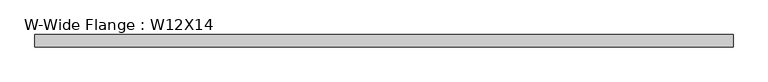
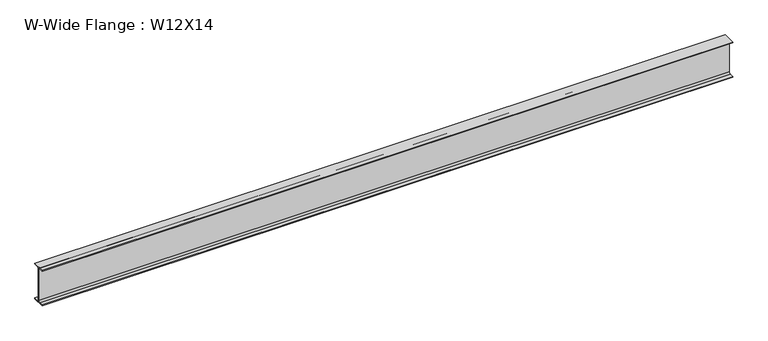
"""IFC4 building model written with IfcOpenShell, lengths in millimetres: beam geometry, W-Wide Flange : W12X14."""

from ifc_helpers import new_model, si_unit, point, frame, frame_2d, origin, place, context, project, spatial, polyline, circle_curve, trimmed, segment, composite_curve, outline, extrude, source, transform, mapped, element, save


def w_wide_flange_w12x14_da603a37(model_context):
    return source(origin(), model_context, "Body", "SweptSolid", [
        extrude(outline(composite_curve([segment(polyline([(50.419, -145.415), (50.419, -151.13), (-50.419, -151.13), (-50.419, -145.415), (-15.875, -145.415)]), True, "CONTINUOUS"), segment(trimmed(circle_curve(frame_2d((-15.875, -132.08)), 13.335), [point((-15.875, -145.415))], [point((-2.54, -132.08))], True, "CARTESIAN"), True, "CONTINUOUS"), segment(polyline([(-2.54, -132.08), (-2.54, 132.08)]), True, "CONTINUOUS"), segment(trimmed(circle_curve(frame_2d((-15.875, 132.08)), 13.335), [point((-2.54, 132.08))], [point((-15.875, 145.415))], True, "CARTESIAN"), True, "CONTINUOUS"), segment(polyline([(-15.875, 145.415), (-50.419, 145.415), (-50.419, 151.13), (50.419, 151.13), (50.419, 145.415), (15.875, 145.415)]), True, "CONTINUOUS"), segment(trimmed(circle_curve(frame_2d((15.875, 132.08)), 13.335), [point((15.875, 145.415))], [point((2.54, 132.08))], True, "CARTESIAN"), True, "CONTINUOUS"), segment(polyline([(2.54, 132.08), (2.54, -132.08)]), True, "CONTINUOUS"), segment(trimmed(circle_curve(frame_2d((15.875, -132.08)), 13.335), [point((2.54, -132.08))], [point((15.875, -145.415))], True, "CARTESIAN"), True, "CONTINUOUS"), segment(polyline([(15.875, -145.415), (50.419, -145.415)]), True, "CONTINUOUS")], self_intersect=False)), frame((-2755.9, 0.0, 0.0), z_axis=(1.0, 0.0, 0.0), x_axis=(0.0, 1.0, 0.0)), (0.0, 0.0, 1.0), 5600.7),
    ])


if __name__ == "__main__":
    model = new_model("IFC4")
    model_context = context("Model", 3, world=origin())
    ifc_project = project(units=[si_unit("LENGTHUNIT", "METRE", prefix="MILLI")], contexts=[model_context])
    site = spatial("IfcSite", under=ifc_project)
    building = spatial("IfcBuilding", under=site)
    placement = place(None, origin())
    w_wide_flange_w12x14_shape = w_wide_flange_w12x14_da603a37(model_context)
    element("IfcBeam", 1, ObjectType="W-Wide Flange : W12X14", at=placement, inside=building, context=model_context, shape_type="MappedRepresentation", body=[
        mapped(w_wide_flange_w12x14_shape, transform((0.0, 0.0, 0.0), x_axis=(1.0, 0.0, 0.0), y_axis=(0.0, 1.0, 0.0), z_axis=(0.0, 0.0, 1.0))),
    ])
    save(model, "model.ifc")

# Revit data of these elements
# Type "W-Wide Flange : W12X14"
#   Assembly Code = "B10"
#   W = 14
#   Length [instance default] = 5' - 0"
#   bf = 0' - 3.97"
#   d = 0' - 11.9"
#   k = 0' - 0 3/4"
#   k2 = 0' - 0.525"
#   tf = 0' - 0.225"
#   tw = 0' - 0.2"
#   A = 0.0288889 SF
#   Structural Material [instance default] = Steel ASTM A992
# Element 1 (IfcBeam, "W-Wide Flange : W12X14")
#   Materials on its faces: "Steel ASTM A992"
# Materials
#   "Steel ASTM A992": class "Metal", colour RGB 199 199 199, transparency 0, Description = "Structural steel 50ksi", Cost = 0
